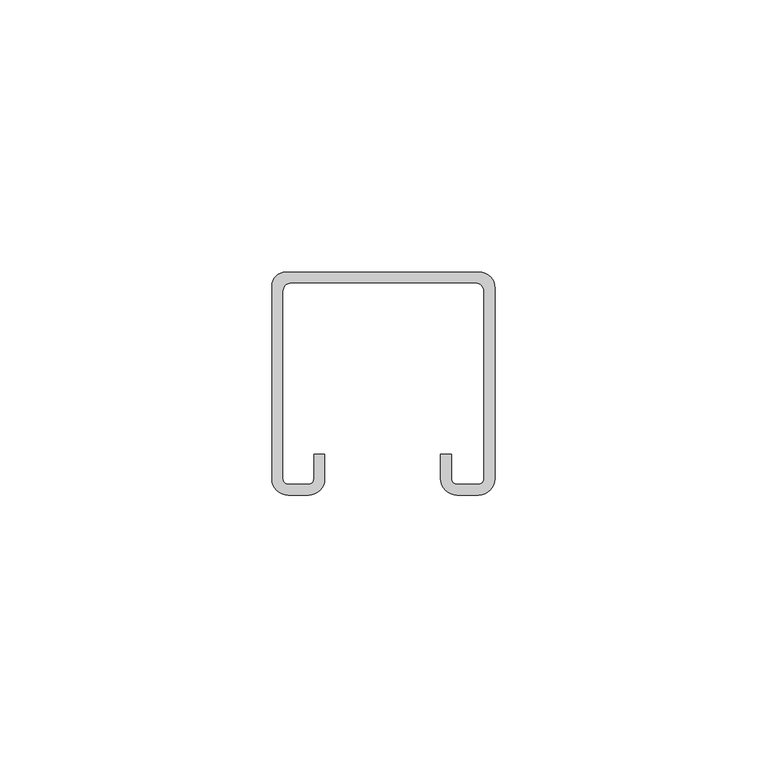
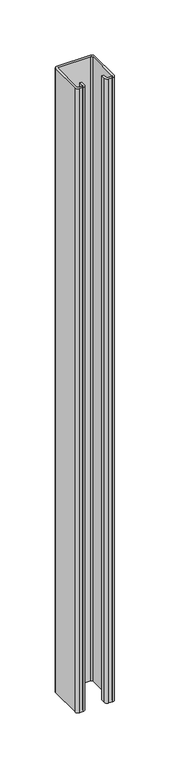
"""IFC4 building model written with IfcOpenShell, lengths in millimetres: proxy geometry, TN_Профиль монтажный : Профиль монтажный 41х41x2,0-3000."""

from ifc_helpers import new_model, si_unit, point, frame_2d, origin, origin_with_axes, place, context, project, spatial, polyline, circle_curve, trimmed, segment, composite_curve, outline, extrude, source, transform, mapped, element, save


def generic_models_fcee67ed(model_context):
    return source(origin(), model_context, "Body", "SweptSolid", [
        extrude(outline(composite_curve([segment(polyline([(20.7157599, -2.9315199), (20.7157599, -38.0)]), True, "CONTINUOUS"), segment(trimmed(circle_curve(frame_2d((17.7157599, -38.0)), 3.0), [point((20.7157599, -38.0))], [point((17.7157599, -41.0))], False, "CARTESIAN"), True, "CONTINUOUS"), segment(polyline([(17.7157599, -41.0), (13.7568638, -41.0)]), True, "CONTINUOUS"), segment(trimmed(circle_curve(frame_2d((13.7568638, -37.9588961)), 3.0411039), [point((13.7568638, -41.0))], [point((10.7157599, -37.9588961))], False, "CARTESIAN"), True, "CONTINUOUS"), segment(polyline([(10.7157599, -37.9588961), (10.7157599, -33.5), (12.7157599, -33.5), (12.7157599, -38.0)]), True, "CONTINUOUS"), segment(trimmed(circle_curve(frame_2d((13.7157599, -38.0)), 1.0), [point((12.7157599, -38.0))], [point((13.7157599, -39.0))], True, "CARTESIAN"), True, "CONTINUOUS"), segment(polyline([(13.7157599, -39.0), (17.7157599, -39.0)]), True, "CONTINUOUS"), segment(trimmed(circle_curve(frame_2d((17.7157599, -38.0)), 1.0), [point((17.7157599, -39.0))], [point((18.7157599, -38.0))], True, "CARTESIAN"), True, "CONTINUOUS"), segment(polyline([(18.7157599, -38.0), (18.7157599, -3.5)]), True, "CONTINUOUS"), segment(trimmed(circle_curve(frame_2d((17.2157599, -3.5)), 1.5), [point((18.7157599, -3.5))], [point((17.2157599, -2.0))], True, "CARTESIAN"), True, "CONTINUOUS"), segment(polyline([(17.2157599, -2.0), (-16.7842401, -2.0)]), True, "CONTINUOUS"), segment(trimmed(circle_curve(frame_2d((-16.7842401, -3.5)), 1.5), [point((-16.7842401, -2.0))], [point((-18.2842401, -3.5))], True, "CARTESIAN"), True, "CONTINUOUS"), segment(polyline([(-18.2842401, -3.5), (-18.2842401, -38.0)]), True, "CONTINUOUS"), segment(trimmed(circle_curve(frame_2d((-17.2842401, -38.0)), 1.0), [point((-18.2842401, -38.0))], [point((-17.2842401, -39.0))], True, "CARTESIAN"), True, "CONTINUOUS"), segment(polyline([(-17.2842401, -39.0), (-13.5684801, -39.0)]), True, "CONTINUOUS"), segment(trimmed(circle_curve(frame_2d((-13.5684801, -38.0)), 1.0), [point((-13.5684801, -39.0))], [point((-12.5684801, -38.0))], True, "CARTESIAN"), True, "CONTINUOUS"), segment(polyline([(-12.5684801, -38.0), (-12.5684801, -33.5), (-10.5684801, -33.5), (-10.5684801, -38.0)]), True, "CONTINUOUS"), segment(trimmed(circle_curve(frame_2d((-13.5684801, -38.0)), 3.0), [point((-10.5684801, -38.0))], [point((-13.5684801, -41.0))], False, "CARTESIAN"), True, "CONTINUOUS"), segment(polyline([(-13.5684801, -41.0), (-17.2842401, -41.0)]), True, "CONTINUOUS"), segment(trimmed(circle_curve(frame_2d((-17.2842401, -38.0)), 3.0), [point((-17.2842401, -41.0))], [point((-20.2842401, -38.0))], False, "CARTESIAN"), True, "CONTINUOUS"), segment(polyline([(-20.2842401, -38.0), (-20.2842401, -2.5)]), True, "CONTINUOUS"), segment(trimmed(circle_curve(frame_2d((-17.7842401, -2.5)), 2.5), [point((-20.2842401, -2.5))], [point((-17.7842401, 0.0))], False, "CARTESIAN"), True, "CONTINUOUS"), segment(polyline([(-17.7842401, 0.0), (17.7842401, 0.0)]), True, "CONTINUOUS"), segment(trimmed(circle_curve(frame_2d((17.7842401, -2.9315199)), 2.9315199), [point((17.7842401, 0.0))], [point((20.7157599, -2.9315199))], False, "CARTESIAN"), True, "CONTINUOUS")], self_intersect=False)), origin_with_axes(), (0.0, 0.0, 1.0), 700.0),
    ])


if __name__ == "__main__":
    model = new_model("IFC4")
    model_context = context("Model", 3, world=origin())
    ifc_project = project(units=[si_unit("LENGTHUNIT", "METRE", prefix="MILLI")], contexts=[model_context])
    site = spatial("IfcSite", under=ifc_project)
    building = spatial("IfcBuilding", under=site)
    placement = place(None, origin())
    generic_models_shape = generic_models_fcee67ed(model_context)
    element("IfcBuildingElementProxy", 1, Name="TN_Профиль монтажный : Профиль монтажный 41х41x2,0-3000", ObjectType="TN_Профиль монтажный : Профиль монтажный 41х41x2,0-3000", at=placement, inside=building, context=model_context, shape_type="MappedRepresentation", body=[
        mapped(generic_models_shape, transform((0.0, 0.0, 0.0), x_axis=(1.0, 0.0, 0.0), y_axis=(0.0, 1.0, 0.0), z_axis=(0.0, 0.0, 1.0))),
    ])
    save(model, "model.ifc")

# Revit data of these elements
# Type "TN_Профиль монтажный : Профиль монтажный 41х41x2,0-3000"
#   Description = "Профиль монтажный – траверса С-образной формы предназначен для горизонтального и вертикального монтажа тяжелых инженерных систем, оборудования систем вентиляции и кондиционирования, установок электроснабжения, элементов трубопроводов, также для изготовления стенных консолей пристенного монтажа, рам оснований различного типа под оборудование. Возможно замещение на основе сконструированных модулей серийных опор ГОСТ для раскрепления технологических трубопроводов. Рекомендуется для применения в сухих, влажных помещениях и на открытом воздухе."
#   Manufacturer = "ТехноНИКОЛЬ"
#   Model = "Комплектующие к опорам"
#   URL = "https://nav.tn.ru/knowledge-base/polimernye-membrany/opory-pod-oborudovanie-na-ploskoy-krovle/?sphrase_id=266812"
#   ADSK_Обозначение = "ТехноНИКОЛЬ"
#   ADSK_Наименование краткое = "П41х41x2,0"
#   ADSK_Наименование = "Профиль монтажный 41х41x2,0-3000"
#   ADSK_Масса_Текст = ""
#   ADSK_Марка = "П41х41x2,0"
#   ADSK_Код изделия = "660816"
#   ADSK_Завод-изготовитель = "ТехноНИКОЛЬ"
#   ADSK_Единица измерения = "п.м."
#   ADSK_Группирование = "Комплектующие к опорам"
#   ADSK_URL страницы изделия = "https://nav.tn.ru/knowledge-base/polimernye-membrany/opory-pod-oborudovanie-na-ploskoy-krovle/?sphrase_id=266812"
#   ADSK_URL документации изделия = ""
#   Размер_Длина_Вводимая [instance default] = 1000 mm
#   ADSK_Размер_Длина [instance default] = 1000 mm
#   ADSK_Количество [instance default] = 1
#   Тип профиля = 1
#   Профиль монтажный 41х41x2,0 = yes
#   Профиль монтажный 41x62x2,5 = no
#   Профиль монтажный 41x124x2,5 = no
#   ADSK_Материал = TN_СтальГальванизированная_Серый
#   Default Elevation = 0
# Element 1 (IfcBuildingElementProxy, "TN_Профиль монтажный : Профиль монтажный 41х41x2,0-3000")
#   Размер_Длина_Вводимая = 700 mm
#   ADSK_Размер_Длина = 700 mm
#   ADSK_Количество = 0.7
#   Materials on its faces: "TN_СтальГальванизированная_Серый"
# Materials
#   "TN_СтальГальванизированная_Серый": class "Типовые", colour RGB 206 210 213, transparency 0, Cost = 0
